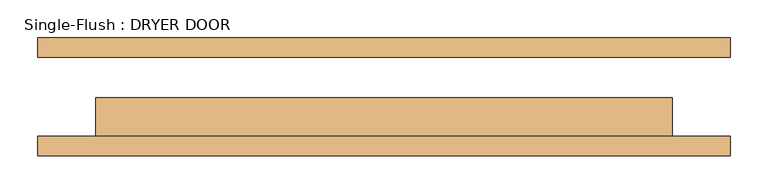
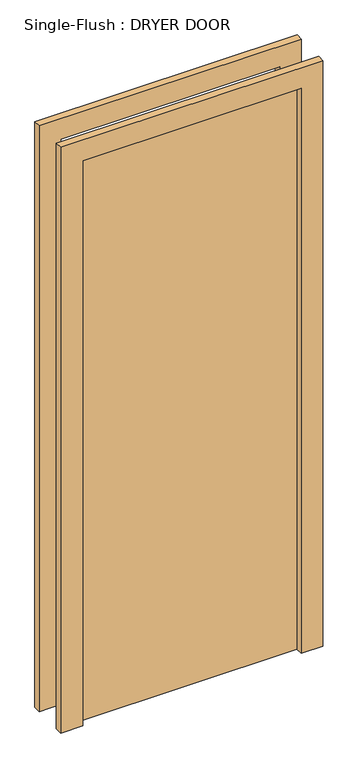
"""IFC4 building model written with IfcOpenShell, lengths in millimetres: door geometry, Single-Flush : DRYER DOOR."""

import ifcopenshell
import ifcopenshell.guid

model = None  # the IFC model being written
_history = None  # IfcOwnerHistory: only IFC2X3 demands one
_inside = {}  # id of a spatial element -> (the spatial element, [elements in it])
_under = {}  # id of a project, library or spatial element -> (it, [spatial elements below it])
_declared = {}  # id of a project -> (the project, [libraries it declares])
_typed = {}  # id of a type object -> (the type object, [elements of that type])
_made_of = {}  # id of a material, layer set ... -> (it, [elements and type objects made of it])


def new_model(schema):
    """Start an empty IFC model of exactly this schema.

    Asked for "IFC4X3", IfcOpenShell would pick the latest addendum, in which some entities
    have other attributes; the version numbers below select the first issue.
    IFC2X3 requires an IfcOwnerHistory on every rooted entity: one is made here for all.
    """
    global model, _history
    if schema == "IFC4X3":
        model = ifcopenshell.file(schema_version=(4, 3, 0, 0))
    else:
        model = ifcopenshell.file(schema=schema)
    _inside.clear()
    _under.clear()
    _declared.clear()
    _typed.clear()
    _made_of.clear()
    _history = None
    if model.schema == "IFC2X3":
        org = make("IfcOrganization", Name="unknown")
        user = make(
            "IfcPersonAndOrganization",
            ThePerson=make("IfcPerson", FamilyName="unknown"),
            TheOrganization=org,
        )
        app = make(
            "IfcApplication",
            ApplicationDeveloper=org,
            Version="unknown",
            ApplicationFullName="unknown",
            ApplicationIdentifier="unknown",
        )
        _history = make(
            "IfcOwnerHistory",
            OwningUser=user,
            OwningApplication=app,
            ChangeAction="ADDED",
            CreationDate=0,
        )
    return model


def make(cls, **values):
    """One entity of the class cls with the attributes given. An attribute that is None is left unset."""
    return model.create_entity(
        cls, **{name: value for name, value in values.items() if value is not None}
    )


def rooted(cls, **values):
    """An entity with a GlobalId (a new one), such as an element, a storey or a relation."""
    return make(cls, GlobalId=ifcopenshell.guid.new(), OwnerHistory=_history, **values)


def si_unit(unit_type, name, prefix=None):
    """IfcSIUnit, for example si_unit("LENGTHUNIT", "METRE", prefix="MILLI")."""
    return make("IfcSIUnit", UnitType=unit_type, Prefix=prefix, Name=name)


def assignment(units):
    """IfcUnitAssignment: the units of a project."""
    return None if units is None else make("IfcUnitAssignment", Units=units)


def point(xyz):
    """IfcCartesianPoint."""
    return None if xyz is None else make("IfcCartesianPoint", Coordinates=xyz)


def direction(xyz):
    """IfcDirection."""
    return None if xyz is None else make("IfcDirection", DirectionRatios=xyz)


def frame(location, z_axis=None, x_axis=None):
    """IfcAxis2Placement3D, a coordinate frame: its origin and axes. An axis left out is left unset."""
    return make(
        "IfcAxis2Placement3D",
        Location=point(location),
        Axis=direction(z_axis),
        RefDirection=direction(x_axis),
    )


def origin():
    """The frame at (0, 0, 0) with its axes left unset."""
    return frame((0.0, 0.0, 0.0))


def origin_with_axes():
    """The frame at (0, 0, 0) with the z axis (0, 0, 1) and the x axis (1, 0, 0) written out."""
    return frame((0.0, 0.0, 0.0), z_axis=(0.0, 0.0, 1.0), x_axis=(1.0, 0.0, 0.0))


def place(relative_to, where):
    """IfcLocalPlacement: puts the frame where relative to a parent placement (None: the world)."""
    return make(
        "IfcLocalPlacement", PlacementRelTo=relative_to, RelativePlacement=where
    )


def context(
    kind, dimensions, precision=None, world=None, true_north=None, identifier=None
):
    """IfcGeometricRepresentationContext, for example the 3D "Model" context."""
    return make(
        "IfcGeometricRepresentationContext",
        ContextIdentifier=identifier,
        ContextType=kind,
        CoordinateSpaceDimension=dimensions,
        Precision=precision,
        WorldCoordinateSystem=world,
        TrueNorth=true_north,
    )


def project(units=None, contexts=None):
    """IfcProject with its units and contexts."""
    return rooted(
        "IfcProject",
        Name="project",
        RepresentationContexts=contexts,
        UnitsInContext=assignment(units),
    )


def spatial(cls, under=None, at=None, **own):
    """A site, building, storey or space (cls), placed at a placement, below another one or the project."""
    s = rooted(cls, ObjectPlacement=at, **own)
    if under is not None:
        _under.setdefault(under.id(), (under, []))[1].append(s)
    return s


def polyline(points):
    """IfcPolyline through the points."""
    return make("IfcPolyline", Points=[point(p) for p in points])


def outline(outer, holes=None, kind="AREA"):
    """IfcArbitraryClosedProfileDef: a profile drawn as a closed curve; with holes, ...WithVoids."""
    if holes is None:
        return make("IfcArbitraryClosedProfileDef", ProfileType=kind, OuterCurve=outer)
    return make(
        "IfcArbitraryProfileDefWithVoids",
        ProfileType=kind,
        OuterCurve=outer,
        InnerCurves=holes,
    )


def extrude(swept, where, along, depth):
    """IfcExtrudedAreaSolid: the profile swept, set in the frame where, extruded along a direction by depth."""
    return make(
        "IfcExtrudedAreaSolid",
        SweptArea=swept,
        Position=where,
        ExtrudedDirection=direction(along),
        Depth=depth,
    )


def shape(context_of_items, identifier, shape_type, items):
    """IfcShapeRepresentation: the items that make up one representation, for example the "Body"."""
    return make(
        "IfcShapeRepresentation",
        ContextOfItems=context_of_items,
        RepresentationIdentifier=identifier,
        RepresentationType=shape_type,
        Items=items,
    )


def source(mapping_origin, context_of_items, identifier, shape_type, items):
    """IfcRepresentationMap: a shape defined once, which mapped items show again and again."""
    return make(
        "IfcRepresentationMap",
        MappingOrigin=mapping_origin,
        MappedRepresentation=shape(context_of_items, identifier, shape_type, items),
    )


def transform(
    local_origin,
    x_axis=None,
    y_axis=None,
    z_axis=None,
    scale=None,
    scale2=None,
    scale3=None,
    uniform=True,
):
    """IfcCartesianTransformationOperator3D, or its non-uniform kind. x_axis, y_axis, z_axis: its Axis1, 2, 3."""
    if uniform:
        return make(
            "IfcCartesianTransformationOperator3D",
            Axis1=direction(x_axis),
            Axis2=direction(y_axis),
            LocalOrigin=point(local_origin),
            Scale=scale,
            Axis3=direction(z_axis),
        )
    return make(
        "IfcCartesianTransformationOperator3DnonUniform",
        Axis1=direction(x_axis),
        Axis2=direction(y_axis),
        LocalOrigin=point(local_origin),
        Scale=scale,
        Axis3=direction(z_axis),
        Scale2=scale2,
        Scale3=scale3,
    )


def mapped(mapping_source, mapping_target):
    """IfcMappedItem: shows the shape of a source again, moved by a transform."""
    return make(
        "IfcMappedItem", MappingSource=mapping_source, MappingTarget=mapping_target
    )


def made_of(thing, what):
    """Note that an element or type object is made of a material, layer set ...; save() writes the relation."""
    if what is not None:
        _made_of.setdefault(what.id(), (what, []))[1].append(thing)
    return thing


def element(
    cls,
    number,
    at=None,
    inside=None,
    cuts=None,
    type_object=None,
    material=None,
    context=None,
    identifier="Body",
    shape_type=None,
    held_by="IfcProductDefinitionShape",
    body=None,
    shapes=None,
    **own,
):
    """One element of the class cls, such as IfcWall. Its Tag is "e" and its number.

    at: its placement. inside: the storey or other place that contains it. cuts: it is an
    opening in that element (IfcRelVoidsElement). A single representation is given by context,
    identifier, shape_type and body (its items); several are given by shapes. held_by: the class
    of the entity that holds the representations. save() writes the other relations.
    """
    e = rooted(cls, Tag="e%d" % number, ObjectPlacement=at, **own)
    if body is not None:
        shapes = [shape(context, identifier, shape_type, body)]
    if shapes is not None:
        e.Representation = make(held_by, Representations=shapes)
    if inside is not None:
        _inside.setdefault(inside.id(), (inside, []))[1].append(e)
    if cuts is not None:
        rooted(
            "IfcRelVoidsElement", RelatingBuildingElement=cuts, RelatedOpeningElement=e
        )
    if type_object is not None:
        _typed.setdefault(type_object.id(), (type_object, []))[1].append(e)
    return made_of(e, material)


def aggregate(whole, parts):
    """IfcRelAggregates: a whole, such as a stair, and the parts it consists of."""
    return rooted("IfcRelAggregates", RelatingObject=whole, RelatedObjects=parts)


def save(model, path):
    """Write the relations noted so far, then the file.

    IfcRelAggregates (storeys below a building ...), IfcRelContainedInSpatialStructure (elements
    in a storey), IfcRelDefinesByType, IfcRelAssociatesMaterial and IfcRelDeclares: one each for
    every whole, place, type object, material and project.
    """
    for whole, parts in _under.values():
        aggregate(whole, parts)
    for where, things in _inside.values():
        rooted(
            "IfcRelContainedInSpatialStructure",
            RelatedElements=things,
            RelatingStructure=where,
        )
    for kind, things in _typed.values():
        rooted("IfcRelDefinesByType", RelatedObjects=things, RelatingType=kind)
    for what, things in _made_of.values():
        rooted("IfcRelAssociatesMaterial", RelatedObjects=things, RelatingMaterial=what)
    for by, libraries in _declared.values():
        rooted("IfcRelDeclares", RelatingContext=by, RelatedDefinitions=libraries)
    model.write(path)


def single_flush_dryer_door_45c3dc5d(model_context):
    return source(origin(), model_context, "Body", "SweptSolid", [
        extrude(outline(polyline([(2159.0, -457.2), (0.0, -457.2), (0.0, -381.0), (2082.8, -381.0), (2082.8, 381.0), (0.0, 381.0), (0.0, 457.2), (2159.0, 457.2), (2159.0, -457.2)])), frame((0.0, -77.7875, 0.0), z_axis=(0.0, 1.0, 0.0), x_axis=(0.0, 0.0, 1.0)), (0.0, 0.0, 1.0), 25.4),
        extrude(outline(polyline([(2159.0, 457.2), (2159.0, -457.2), (0.0, -457.2), (0.0, -381.0), (2082.8, -381.0), (2082.8, 381.0), (0.0, 381.0), (0.0, 457.2), (2159.0, 457.2)])), frame((0.0, 52.3875, 0.0), z_axis=(0.0, 1.0, 0.0), x_axis=(0.0, 0.0, 1.0)), (0.0, 0.0, 1.0), 25.4),
        extrude(outline(polyline([(381.0, -1.5875), (381.0, -52.3875), (-381.0, -52.3875), (-381.0, -1.5875), (381.0, -1.5875)])), origin_with_axes(), (0.0, 0.0, 1.0), 2082.8),
    ])


if __name__ == "__main__":
    model = new_model("IFC4")
    model_context = context("Model", 3, world=origin())
    ifc_project = project(units=[si_unit("LENGTHUNIT", "METRE", prefix="MILLI")], contexts=[model_context])
    site = spatial("IfcSite", under=ifc_project)
    building = spatial("IfcBuilding", under=site)
    placement = place(None, origin())
    single_flush_dryer_door_shape = single_flush_dryer_door_45c3dc5d(model_context)
    element("IfcDoor", 1, ObjectType="Single-Flush : DRYER DOOR", at=placement, inside=building, context=model_context, shape_type="MappedRepresentation", body=[
        mapped(single_flush_dryer_door_shape, transform((0.0, 0.0, 0.0), x_axis=(1.0, 0.0, 0.0), y_axis=(0.0, 1.0, 0.0), z_axis=(0.0, 0.0, 1.0))),
    ])
    save(model, "model.ifc")

# Revit data of these elements
# Type "Single-Flush : DRYER DOOR"
#   Type Mark = "01"
#   Assembly Code = "C1020"
#   Thickness = 0' - 2"
#   Height = 6' - 10"
#   Trim Projection Ext = 0' - 1"
#   Trim Projection Int = 0' - 1"
#   Trim Width = 0' - 3"
#   Width = 2' - 6"
#   Door Material = EXISTING WALL (SHADED)
#   Frame Material = EXISTING WALL (SHADED)
#   Function = (empty or 0)
#   Wall Closure = (empty or 0)
# Element 1 (IfcDoor, "Single-Flush : DRYER DOOR")
#   Materials on its faces: "EXISTING WALL (SHADED)"
# Materials
#   "EXISTING WALL (SHADED)": class "Generic", colour RGB 255 255 255, transparency 0, Cost = 0
